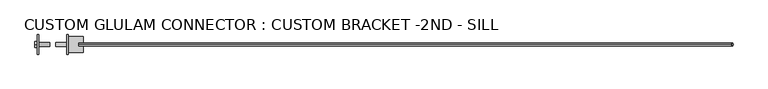
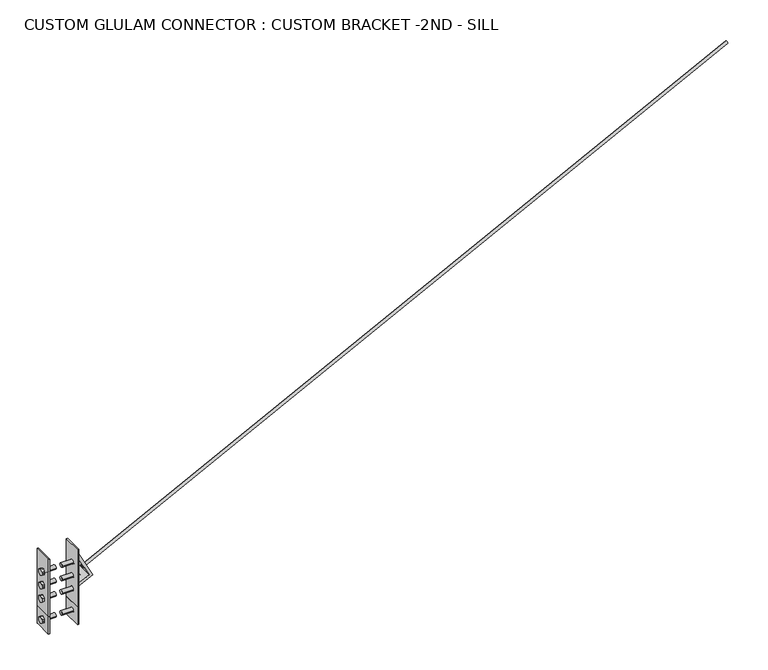
"""IFC4 building model written with IfcOpenShell, lengths in millimetres: fastener geometry, CUSTOM GLULAM CONNECTOR : CUSTOM BRACKET -2ND - SILL."""

from ifc_helpers import new_model, si_unit, point, frame, frame_2d, origin, place, context, project, spatial, polyline, circle_curve, trimmed, segment, composite_curve, outline, extrude, source, transform, mapped, element, save
from ifc_brep_helpers import plane_surface, revolved_surface, advanced_brep


def custom_glulam_connector_custom_bracket_2nd_sill_58b813d6(model_context):
    return source(origin(), model_context, "Body", "SolidModel", [
        advanced_brep(
        [(-95.25, -60.325, 122.2375), (-87.3125, -60.325, 122.2375), (-87.3125, 60.325, 122.2375), (-95.25, 60.325, 122.2375), (-95.25, 52.3875, 122.2375), (-95.25, -60.325, 7.9375), (-87.3125, -60.325, 7.9375), (-95.25, -13.890625, 71.4375), (-95.25, 13.890625, 71.4375), (-87.3125, 13.890625, 71.4375), (-87.3125, -13.890625, 71.4375), (-95.25, 60.325, 7.9375), (-95.25, 52.3875, 7.9375), (-87.3125, 60.325, 7.9375)],
        [
            (0, 1),
            (1, 2),
            (2, 3),
            (3, 4),
            (4, 0),
            (5, 6),
            (6, 1),
            (0, 5),
            (7, 8, circle_curve(frame((-95.25, 0.0, 71.4375), z_axis=(-1.0, 0.0, 0.0), x_axis=(0.0, 1.0, 0.0)), 13.890625)),
            (8, 9),
            (9, 10, circle_curve(frame((-87.3125, 0.0, 71.4375), z_axis=(1.0, 0.0, 0.0), x_axis=(0.0, 1.0, 0.0)), 13.890625)),
            (10, 7),
            (3, 11),
            (11, 12),
            (12, 5),
            (7, 8, circle_curve(frame((-95.25, 0.0, 71.4375), z_axis=(1.0, 0.0, 0.0), x_axis=(0.0, 1.0, 0.0)), 13.890625)),
            (2, 13),
            (13, 11),
            (10, 9, circle_curve(frame((-87.3125, 0.0, 71.4375), z_axis=(1.0, 0.0, 0.0), x_axis=(0.0, 1.0, 0.0)), 13.890625)),
            (6, 13),
        ],
        [
            plane_surface(frame((-95.25, 60.325, 122.2375), z_axis=(0.0, 0.0, 1.0), x_axis=(1.0, 0.0, 0.0))),
            plane_surface(frame((-95.25, -60.325, 122.2375), z_axis=(0.0, -1.0, 0.0), x_axis=(1.0, 0.0, 0.0))),
            revolved_surface(polyline([(-95.25, 13.890625, 71.4375), (-87.3125, 13.890625, 71.4375)]), (-87.3125, 0.0, 71.4375), (-1.0, 0.0, 0.0)),
            plane_surface(frame((-95.25, -60.325, 122.2375), z_axis=(-1.0, 0.0, 0.0), x_axis=(0.0, -1.0, 0.0))),
            plane_surface(frame((-95.25, 60.325, 7.9375), z_axis=(0.0, 1.0, 0.0), x_axis=(1.0, 0.0, 0.0))),
            plane_surface(frame((-87.3125, -60.325, 122.2375), z_axis=(1.0, 0.0, 0.0), x_axis=(0.0, 1.0, 0.0))),
            plane_surface(frame((-95.25, -60.325, 7.9375), z_axis=(0.0, 0.0, -1.0), x_axis=(1.0, 0.0, 0.0))),
        ],
        [
            (0, [[1, 2, 3, 4, 5]]),
            (1, [[6, 7, -1, 8]]),
            (2, [[9, 10, 11, 12]]),
            (3, [[13, 14, 15, -8, -5, -4], [-9, 16]]),
            (4, [[-3, 17, 18, -13]]),
            (2, [[19, -10, -16, -12]]),
            (5, [[-2, -7, 20, -17], [-11, -19]]),
            (6, [[-18, -20, -6, -15, -14]]),
        ],
    ),
        extrude(outline(polyline([(-19.05, 82.4360226), (0.0, 93.4345453), (19.05, 82.4360226), (19.05, 60.4389774), (0.0, 49.4404547), (-19.05, 60.4389774), (-19.05, 82.4360226)])), frame((-110.2320312, 0.0, 0.0), z_axis=(1.0, 0.0, 0.0), x_axis=(0.0, 1.0, 0.0)), (0.0, 0.0, 1.0), 14.9820312),
        extrude(outline(composite_curve([segment(trimmed(circle_curve(frame_2d((0.0, 71.4375)), 12.7), [point((-12.7, 71.4375))], [point((12.7, 71.4375))], False, "CARTESIAN"), True, "CONTINUOUS"), segment(trimmed(circle_curve(frame_2d((0.0, 71.4375)), 12.7), [point((12.7, 71.4375))], [point((-12.7, 71.4375))], False, "CARTESIAN"), True, "CONTINUOUS")], self_intersect=False)), frame((-95.25, 0.0, 0.0), z_axis=(1.0, 0.0, 0.0), x_axis=(0.0, 1.0, 0.0)), (0.0, 0.0, 1.0), 76.2),
        advanced_brep(
        [(95.25, -60.325, 122.2375), (95.25, 52.3875, 122.2375), (95.25, 60.325, 122.2375), (87.3125, 60.325, 122.2375), (87.3125, -60.325, 122.2375), (95.25, -60.325, 7.9375), (87.3125, -60.325, 7.9375), (95.25, -13.890625, 71.4375), (87.3125, -13.890625, 71.4375), (87.3125, 13.890625, 71.4375), (95.25, 13.890625, 71.4375), (95.25, 52.3875, 7.9375), (95.25, 60.325, 7.9375), (87.3125, 60.325, 7.9375)],
        [
            (0, 1),
            (1, 2),
            (2, 3),
            (3, 4),
            (4, 0),
            (5, 0),
            (4, 6),
            (6, 5),
            (7, 8),
            (8, 9, circle_curve(frame((87.3125, 0.0, 71.4375), z_axis=(-1.0, 0.0, 0.0), x_axis=(0.0, 1.0, 0.0)), 13.890625)),
            (9, 10),
            (10, 7, circle_curve(frame((95.25, 0.0, 71.4375), z_axis=(1.0, 0.0, 0.0), x_axis=(0.0, 1.0, 0.0)), 13.890625)),
            (5, 11),
            (11, 12),
            (12, 2),
            (10, 7, circle_curve(frame((95.25, 0.0, 71.4375), z_axis=(-1.0, 0.0, 0.0), x_axis=(0.0, 1.0, 0.0)), 13.890625)),
            (12, 13),
            (13, 3),
            (9, 8, circle_curve(frame((87.3125, 0.0, 71.4375), z_axis=(-1.0, 0.0, 0.0), x_axis=(0.0, 1.0, 0.0)), 13.890625)),
            (13, 6),
        ],
        [
            plane_surface(frame((95.25, 60.325, 122.2375), z_axis=(0.0, 0.0, 1.0), x_axis=(-1.0, 0.0, 0.0))),
            plane_surface(frame((95.25, -60.325, 122.2375), z_axis=(0.0, -1.0, 0.0), x_axis=(-1.0, 0.0, 0.0))),
            revolved_surface(polyline([(95.25, 13.890625, 71.4375), (87.3125, 13.890625, 71.4375)]), (87.3125, 0.0, 71.4375), (1.0, 0.0, 0.0)),
            plane_surface(frame((95.25, -60.325, 122.2375), z_axis=(1.0, 0.0, 0.0), x_axis=(0.0, -1.0, 0.0))),
            plane_surface(frame((95.25, 60.325, 7.9375), z_axis=(0.0, 1.0, 0.0), x_axis=(-1.0, 0.0, 0.0))),
            plane_surface(frame((87.3125, -60.325, 122.2375), z_axis=(-1.0, 0.0, 0.0), x_axis=(0.0, 1.0, 0.0))),
            plane_surface(frame((95.25, -60.325, 7.9375), z_axis=(0.0, 0.0, -1.0), x_axis=(-1.0, 0.0, 0.0))),
        ],
        [
            (0, [[1, 2, 3, 4, 5]]),
            (1, [[6, -5, 7, 8]]),
            (2, [[9, 10, 11, 12]]),
            (3, [[-2, -1, -6, 13, 14, 15], [16, -12]]),
            (4, [[-15, 17, 18, -3]]),
            (2, [[-9, -16, -11, 19]]),
            (5, [[-18, 20, -7, -4], [-19, -10]]),
            (6, [[-14, -13, -8, -20, -17]]),
        ],
    ),
        extrude(outline(polyline([(-19.05, 82.4360226), (0.0, 93.4345453), (19.05, 82.4360226), (19.05, 60.4389774), (0.0, 49.4404547), (-19.05, 60.4389774), (-19.05, 82.4360226)])), frame((95.25, 0.0, 0.0), z_axis=(1.0, 0.0, 0.0), x_axis=(0.0, 1.0, 0.0)), (0.0, 0.0, 1.0), 14.9820312),
        extrude(outline(composite_curve([segment(trimmed(circle_curve(frame_2d((0.0, 71.4375)), 12.7), [point((-12.7, 71.4375))], [point((12.7, 71.4375))], False, "CARTESIAN"), True, "CONTINUOUS"), segment(trimmed(circle_curve(frame_2d((0.0, 71.4375)), 12.7), [point((12.7, 71.4375))], [point((-12.7, 71.4375))], False, "CARTESIAN"), True, "CONTINUOUS")], self_intersect=False)), frame((19.05, 0.0, 0.0), z_axis=(1.0, 0.0, 0.0), x_axis=(0.0, 1.0, 0.0)), (0.0, 0.0, 1.0), 76.2),
        advanced_brep(
        [(-95.25, 60.325, 503.2375), (-87.3125, 60.325, 503.2375), (-87.3125, 60.325, 122.2375), (-95.25, 60.325, 122.2375), (-87.3125, -13.890625, 388.9375), (-87.3125, 13.890625, 388.9375), (-95.25, 13.890625, 388.9375), (-95.25, -13.890625, 388.9375), (-95.25, -60.325, 503.2375), (-87.3125, -60.325, 503.2375), (-95.25, -52.3875, 503.2375), (-95.25, -52.3875, 122.2375), (-95.25, -60.325, 122.2375), (-95.25, 13.890625, 300.0375), (-95.25, -13.890625, 300.0375), (-95.25, 13.890625, 211.1375), (-95.25, -13.890625, 211.1375), (-87.3125, -13.890625, 300.0375), (-87.3125, 13.890625, 300.0375), (-87.3125, -60.325, 122.2375), (-87.3125, -13.890625, 211.1375), (-87.3125, 13.890625, 211.1375)],
        [
            (0, 1),
            (1, 2),
            (2, 3),
            (3, 0),
            (4, 5, circle_curve(frame((-87.3125, 0.0, 388.9375), z_axis=(1.0, 0.0, 0.0), x_axis=(0.0, 1.0, 0.0)), 13.890625)),
            (5, 6),
            (6, 7, circle_curve(frame((-95.25, 0.0, 388.9375), z_axis=(-1.0, 0.0, 0.0), x_axis=(0.0, 1.0, 0.0)), 13.890625)),
            (7, 4),
            (7, 6, circle_curve(frame((-95.25, 0.0, 388.9375), z_axis=(-1.0, 0.0, 0.0), x_axis=(0.0, 1.0, 0.0)), 13.890625)),
            (5, 4, circle_curve(frame((-87.3125, 0.0, 388.9375), z_axis=(1.0, 0.0, 0.0), x_axis=(0.0, 1.0, 0.0)), 13.890625)),
            (8, 9),
            (9, 1),
            (0, 10),
            (10, 8),
            (3, 11),
            (11, 12),
            (12, 8),
            (13, 14, circle_curve(frame((-95.25, 0.0, 300.0375), z_axis=(1.0, 0.0, 0.0), x_axis=(0.0, 1.0, 0.0)), 13.890625)),
            (14, 13, circle_curve(frame((-95.25, 0.0, 300.0375), z_axis=(1.0, 0.0, 0.0), x_axis=(0.0, 1.0, 0.0)), 13.890625)),
            (15, 16, circle_curve(frame((-95.25, 0.0, 211.1375), z_axis=(1.0, 0.0, 0.0), x_axis=(0.0, 1.0, 0.0)), 13.890625)),
            (16, 15, circle_curve(frame((-95.25, 0.0, 211.1375), z_axis=(1.0, 0.0, 0.0), x_axis=(0.0, 1.0, 0.0)), 13.890625)),
            (17, 18, circle_curve(frame((-87.3125, 0.0, 300.0375), z_axis=(1.0, 0.0, 0.0), x_axis=(0.0, 1.0, 0.0)), 13.890625)),
            (18, 13),
            (14, 17),
            (18, 17, circle_curve(frame((-87.3125, 0.0, 300.0375), z_axis=(1.0, 0.0, 0.0), x_axis=(0.0, 1.0, 0.0)), 13.890625)),
            (9, 19),
            (19, 2),
            (20, 21, circle_curve(frame((-87.3125, 0.0, 211.1375), z_axis=(-1.0, 0.0, 0.0), x_axis=(0.0, 1.0, 0.0)), 13.890625)),
            (21, 20, circle_curve(frame((-87.3125, 0.0, 211.1375), z_axis=(-1.0, 0.0, 0.0), x_axis=(0.0, 1.0, 0.0)), 13.890625)),
            (12, 19),
            (21, 15),
            (16, 20),
        ],
        [
            plane_surface(frame((-95.25, 60.325, 122.2375), z_axis=(0.0, 1.0, 0.0), x_axis=(1.0, 0.0, 0.0))),
            revolved_surface(polyline([(-95.25, 13.890625, 388.9375), (-87.3125, 13.890625, 388.9375)]), (-87.3125, 0.0, 388.9375), (-1.0, 0.0, 0.0)),
            plane_surface(frame((-95.25, 60.325, 503.2375), z_axis=(0.0, 0.0, 1.0), x_axis=(1.0, 0.0, 0.0))),
            plane_surface(frame((-95.25, -60.325, 503.2375), z_axis=(-1.0, 0.0, 0.0), x_axis=(0.0, -1.0, 0.0))),
            revolved_surface(polyline([(-95.25, 13.890625, 300.0375), (-87.3125, 13.890625, 300.0375)]), (-87.3125, 0.0, 300.0375), (-1.0, 0.0, 0.0)),
            plane_surface(frame((-87.3125, -60.325, 503.2375), z_axis=(1.0, 0.0, 0.0), x_axis=(0.0, 1.0, 0.0))),
            plane_surface(frame((-95.25, -60.325, 503.2375), z_axis=(0.0, -1.0, 0.0), x_axis=(1.0, 0.0, 0.0))),
            plane_surface(frame((-95.25, -60.325, 122.2375), z_axis=(0.0, 0.0, -1.0), x_axis=(1.0, 0.0, 0.0))),
            revolved_surface(polyline([(-95.25, 13.890625, 211.1375), (-87.3125, 13.890625, 211.1375)]), (-87.3125, 0.0, 211.1375), (-1.0, 0.0, 0.0)),
        ],
        [
            (0, [[1, 2, 3, 4]]),
            (1, [[5, 6, 7, 8]]),
            (1, [[9, -6, 10, -8]]),
            (2, [[11, 12, -1, 13, 14]]),
            (3, [[-4, 15, 16, 17, -14, -13], [18, 19], [-9, -7], [20, 21]]),
            (4, [[22, 23, -19, 24]]),
            (4, [[-18, -23, 25, -24]]),
            (5, [[-12, 26, 27, -2], [-10, -5], [-25, -22], [28, 29]]),
            (6, [[30, -26, -11, -17]]),
            (7, [[-3, -27, -30, -16, -15]]),
            (8, [[-29, 31, -21, 32]]),
            (8, [[-20, -31, -28, -32]]),
        ],
    ),
        extrude(outline(polyline([(-19.05, 399.9360226), (0.0, 410.9345453), (19.05, 399.9360226), (19.05, 377.9389774), (0.0, 366.9404547), (-19.05, 377.9389774), (-19.05, 399.9360226)])), frame((-110.2320312, 0.0, 0.0), z_axis=(1.0, 0.0, 0.0), x_axis=(0.0, 1.0, 0.0)), (0.0, 0.0, 1.0), 14.9820312),
        extrude(outline(composite_curve([segment(trimmed(circle_curve(frame_2d((0.0, 388.9375)), 12.7), [point((-12.7, 388.9375))], [point((12.7, 388.9375))], False, "CARTESIAN"), True, "CONTINUOUS"), segment(trimmed(circle_curve(frame_2d((0.0, 388.9375)), 12.7), [point((12.7, 388.9375))], [point((-12.7, 388.9375))], False, "CARTESIAN"), True, "CONTINUOUS")], self_intersect=False)), frame((-95.25, 0.0, 0.0), z_axis=(1.0, 0.0, 0.0), x_axis=(0.0, 1.0, 0.0)), (0.0, 0.0, 1.0), 76.2),
        extrude(outline(polyline([(-19.05, 311.0360226), (0.0, 322.0345453), (19.05, 311.0360226), (19.05, 289.0389774), (0.0, 278.0404547), (-19.05, 289.0389774), (-19.05, 311.0360226)])), frame((-110.2320312, 0.0, 0.0), z_axis=(1.0, 0.0, 0.0), x_axis=(0.0, 1.0, 0.0)), (0.0, 0.0, 1.0), 14.9820312),
        extrude(outline(composite_curve([segment(trimmed(circle_curve(frame_2d((0.0, 300.0375)), 12.7), [point((-12.7, 300.0375))], [point((12.7, 300.0375))], False, "CARTESIAN"), True, "CONTINUOUS"), segment(trimmed(circle_curve(frame_2d((0.0, 300.0375)), 12.7), [point((12.7, 300.0375))], [point((-12.7, 300.0375))], False, "CARTESIAN"), True, "CONTINUOUS")], self_intersect=False)), frame((-95.25, 0.0, 0.0), z_axis=(1.0, 0.0, 0.0), x_axis=(0.0, 1.0, 0.0)), (0.0, 0.0, 1.0), 76.2),
        extrude(outline(polyline([(-19.05, 399.9360226), (0.0, 410.9345453), (19.05, 399.9360226), (19.05, 377.9389774), (0.0, 366.9404547), (-19.05, 377.9389774), (-19.05, 399.9360226)])), frame((-110.2320312, 0.0, 0.0), z_axis=(1.0, 0.0, 0.0), x_axis=(0.0, 1.0, 0.0)), (0.0, 0.0, 1.0), 14.9820312),
        extrude(outline(composite_curve([segment(trimmed(circle_curve(frame_2d((0.0, 388.9375)), 12.7), [point((-12.7, 388.9375))], [point((12.7, 388.9375))], False, "CARTESIAN"), True, "CONTINUOUS"), segment(trimmed(circle_curve(frame_2d((0.0, 388.9375)), 12.7), [point((12.7, 388.9375))], [point((-12.7, 388.9375))], False, "CARTESIAN"), True, "CONTINUOUS")], self_intersect=False)), frame((-95.25, 0.0, 0.0), z_axis=(1.0, 0.0, 0.0), x_axis=(0.0, 1.0, 0.0)), (0.0, 0.0, 1.0), 76.2),
        extrude(outline(polyline([(-19.05, 222.1360226), (0.0, 233.1345453), (19.05, 222.1360226), (19.05, 200.1389774), (0.0, 189.1404547), (-19.05, 200.1389774), (-19.05, 222.1360226)])), frame((-110.2320312, 0.0, 0.0), z_axis=(1.0, 0.0, 0.0), x_axis=(0.0, 1.0, 0.0)), (0.0, 0.0, 1.0), 14.9820312),
        extrude(outline(composite_curve([segment(trimmed(circle_curve(frame_2d((0.0, 211.1375)), 12.7), [point((-12.7, 211.1375))], [point((12.7, 211.1375))], False, "CARTESIAN"), True, "CONTINUOUS"), segment(trimmed(circle_curve(frame_2d((0.0, 211.1375)), 12.7), [point((12.7, 211.1375))], [point((-12.7, 211.1375))], False, "CARTESIAN"), True, "CONTINUOUS")], self_intersect=False)), frame((-95.25, 0.0, 0.0), z_axis=(1.0, 0.0, 0.0), x_axis=(0.0, 1.0, 0.0)), (0.0, 0.0, 1.0), 76.2),
        advanced_brep(
        [(95.25, 60.325, 503.2375), (95.25, 60.325, 122.2375), (87.3125, 60.325, 122.2375), (87.3125, 60.325, 503.2375), (87.3125, -13.890625, 388.9375), (95.25, -13.890625, 388.9375), (95.25, 13.890625, 388.9375), (87.3125, 13.890625, 388.9375), (95.25, -60.325, 503.2375), (95.25, -52.3875, 503.2375), (87.3125, -60.325, 503.2375), (95.25, -60.325, 122.2375), (95.25, -52.3875, 122.2375), (95.25, 13.890625, 300.0375), (95.25, -13.890625, 300.0375), (95.25, 13.890625, 211.1375), (95.25, -13.890625, 211.1375), (87.3125, -13.890625, 300.0375), (87.3125, 13.890625, 300.0375), (87.3125, -60.325, 122.2375), (87.3125, -13.890625, 211.1375), (87.3125, 13.890625, 211.1375)],
        [
            (0, 1),
            (1, 2),
            (2, 3),
            (3, 0),
            (4, 5),
            (5, 6, circle_curve(frame((95.25, 0.0, 388.9375), z_axis=(1.0, 0.0, 0.0), x_axis=(0.0, 1.0, 0.0)), 13.890625)),
            (6, 7),
            (7, 4, circle_curve(frame((87.3125, 0.0, 388.9375), z_axis=(-1.0, 0.0, 0.0), x_axis=(0.0, 1.0, 0.0)), 13.890625)),
            (4, 7, circle_curve(frame((87.3125, 0.0, 388.9375), z_axis=(-1.0, 0.0, 0.0), x_axis=(0.0, 1.0, 0.0)), 13.890625)),
            (6, 5, circle_curve(frame((95.25, 0.0, 388.9375), z_axis=(1.0, 0.0, 0.0), x_axis=(0.0, 1.0, 0.0)), 13.890625)),
            (8, 9),
            (9, 0),
            (3, 10),
            (10, 8),
            (8, 11),
            (11, 12),
            (12, 1),
            (13, 14, circle_curve(frame((95.25, 0.0, 300.0375), z_axis=(-1.0, 0.0, 0.0), x_axis=(0.0, 1.0, 0.0)), 13.890625)),
            (14, 13, circle_curve(frame((95.25, 0.0, 300.0375), z_axis=(-1.0, 0.0, 0.0), x_axis=(0.0, 1.0, 0.0)), 13.890625)),
            (15, 16, circle_curve(frame((95.25, 0.0, 211.1375), z_axis=(-1.0, 0.0, 0.0), x_axis=(0.0, 1.0, 0.0)), 13.890625)),
            (16, 15, circle_curve(frame((95.25, 0.0, 211.1375), z_axis=(-1.0, 0.0, 0.0), x_axis=(0.0, 1.0, 0.0)), 13.890625)),
            (17, 14),
            (13, 18),
            (18, 17, circle_curve(frame((87.3125, 0.0, 300.0375), z_axis=(-1.0, 0.0, 0.0), x_axis=(0.0, 1.0, 0.0)), 13.890625)),
            (17, 18, circle_curve(frame((87.3125, 0.0, 300.0375), z_axis=(-1.0, 0.0, 0.0), x_axis=(0.0, 1.0, 0.0)), 13.890625)),
            (2, 19),
            (19, 10),
            (20, 21, circle_curve(frame((87.3125, 0.0, 211.1375), z_axis=(1.0, 0.0, 0.0), x_axis=(0.0, 1.0, 0.0)), 13.890625)),
            (21, 20, circle_curve(frame((87.3125, 0.0, 211.1375), z_axis=(1.0, 0.0, 0.0), x_axis=(0.0, 1.0, 0.0)), 13.890625)),
            (19, 11),
            (20, 16),
            (15, 21),
        ],
        [
            plane_surface(frame((95.25, 60.325, 122.2375), z_axis=(0.0, 1.0, 0.0), x_axis=(-1.0, 0.0, 0.0))),
            revolved_surface(polyline([(95.25, 13.890625, 388.9375), (87.3125, 13.890625, 388.9375)]), (87.3125, 0.0, 388.9375), (1.0, 0.0, 0.0)),
            plane_surface(frame((95.25, 60.325, 503.2375), z_axis=(0.0, 0.0, 1.0), x_axis=(-1.0, 0.0, 0.0))),
            plane_surface(frame((95.25, -60.325, 503.2375), z_axis=(1.0, 0.0, 0.0), x_axis=(0.0, -1.0, 0.0))),
            revolved_surface(polyline([(95.25, 13.890625, 300.0375), (87.3125, 13.890625, 300.0375)]), (87.3125, 0.0, 300.0375), (1.0, 0.0, 0.0)),
            plane_surface(frame((87.3125, -60.325, 503.2375), z_axis=(-1.0, 0.0, 0.0), x_axis=(0.0, 1.0, 0.0))),
            plane_surface(frame((95.25, -60.325, 503.2375), z_axis=(0.0, -1.0, 0.0), x_axis=(-1.0, 0.0, 0.0))),
            plane_surface(frame((95.25, -60.325, 122.2375), z_axis=(0.0, 0.0, -1.0), x_axis=(-1.0, 0.0, 0.0))),
            revolved_surface(polyline([(95.25, 13.890625, 211.1375), (87.3125, 13.890625, 211.1375)]), (87.3125, 0.0, 211.1375), (1.0, 0.0, 0.0)),
        ],
        [
            (0, [[1, 2, 3, 4]]),
            (1, [[5, 6, 7, 8]]),
            (1, [[-5, 9, -7, 10]]),
            (2, [[11, 12, -4, 13, 14]]),
            (3, [[-12, -11, 15, 16, 17, -1], [-6, -10], [18, 19], [20, 21]]),
            (4, [[22, -18, 23, 24]]),
            (4, [[-22, 25, -23, -19]]),
            (5, [[-3, 26, 27, -13], [-8, -9], [-24, -25], [28, 29]]),
            (6, [[-15, -14, -27, 30]]),
            (7, [[-17, -16, -30, -26, -2]]),
            (8, [[31, -20, 32, -28]]),
            (8, [[-31, -29, -32, -21]]),
        ],
    ),
        extrude(outline(polyline([(-19.05, 399.9360226), (0.0, 410.9345453), (19.05, 399.9360226), (19.05, 377.9389774), (0.0, 366.9404547), (-19.05, 377.9389774), (-19.05, 399.9360226)])), frame((95.25, 0.0, 0.0), z_axis=(1.0, 0.0, 0.0), x_axis=(0.0, 1.0, 0.0)), (0.0, 0.0, 1.0), 14.9820312),
        extrude(outline(composite_curve([segment(trimmed(circle_curve(frame_2d((0.0, 388.9375)), 12.7), [point((-12.7, 388.9375))], [point((12.7, 388.9375))], False, "CARTESIAN"), True, "CONTINUOUS"), segment(trimmed(circle_curve(frame_2d((0.0, 388.9375)), 12.7), [point((12.7, 388.9375))], [point((-12.7, 388.9375))], False, "CARTESIAN"), True, "CONTINUOUS")], self_intersect=False)), frame((19.05, 0.0, 0.0), z_axis=(1.0, 0.0, 0.0), x_axis=(0.0, 1.0, 0.0)), (0.0, 0.0, 1.0), 76.2),
        extrude(outline(polyline([(-19.05, 311.0360226), (0.0, 322.0345453), (19.05, 311.0360226), (19.05, 289.0389774), (0.0, 278.0404547), (-19.05, 289.0389774), (-19.05, 311.0360226)])), frame((95.25, 0.0, 0.0), z_axis=(1.0, 0.0, 0.0), x_axis=(0.0, 1.0, 0.0)), (0.0, 0.0, 1.0), 14.9820312),
        extrude(outline(composite_curve([segment(trimmed(circle_curve(frame_2d((0.0, 300.0375)), 12.7), [point((-12.7, 300.0375))], [point((12.7, 300.0375))], False, "CARTESIAN"), True, "CONTINUOUS"), segment(trimmed(circle_curve(frame_2d((0.0, 300.0375)), 12.7), [point((12.7, 300.0375))], [point((-12.7, 300.0375))], False, "CARTESIAN"), True, "CONTINUOUS")], self_intersect=False)), frame((19.05, 0.0, 0.0), z_axis=(1.0, 0.0, 0.0), x_axis=(0.0, 1.0, 0.0)), (0.0, 0.0, 1.0), 76.2),
        extrude(outline(polyline([(-19.05, 399.9360226), (0.0, 410.9345453), (19.05, 399.9360226), (19.05, 377.9389774), (0.0, 366.9404547), (-19.05, 377.9389774), (-19.05, 399.9360226)])), frame((95.25, 0.0, 0.0), z_axis=(1.0, 0.0, 0.0), x_axis=(0.0, 1.0, 0.0)), (0.0, 0.0, 1.0), 14.9820312),
        extrude(outline(composite_curve([segment(trimmed(circle_curve(frame_2d((0.0, 388.9375)), 12.7), [point((-12.7, 388.9375))], [point((12.7, 388.9375))], False, "CARTESIAN"), True, "CONTINUOUS"), segment(trimmed(circle_curve(frame_2d((0.0, 388.9375)), 12.7), [point((12.7, 388.9375))], [point((-12.7, 388.9375))], False, "CARTESIAN"), True, "CONTINUOUS")], self_intersect=False)), frame((19.05, 0.0, 0.0), z_axis=(1.0, 0.0, 0.0), x_axis=(0.0, 1.0, 0.0)), (0.0, 0.0, 1.0), 76.2),
        extrude(outline(polyline([(-19.05, 222.1360226), (0.0, 233.1345453), (19.05, 222.1360226), (19.05, 200.1389774), (0.0, 189.1404547), (-19.05, 200.1389774), (-19.05, 222.1360226)])), frame((95.25, 0.0, 0.0), z_axis=(1.0, 0.0, 0.0), x_axis=(0.0, 1.0, 0.0)), (0.0, 0.0, 1.0), 14.9820312),
        extrude(outline(composite_curve([segment(trimmed(circle_curve(frame_2d((0.0, 211.1375)), 12.7), [point((-12.7, 211.1375))], [point((12.7, 211.1375))], False, "CARTESIAN"), True, "CONTINUOUS"), segment(trimmed(circle_curve(frame_2d((0.0, 211.1375)), 12.7), [point((12.7, 211.1375))], [point((-12.7, 211.1375))], False, "CARTESIAN"), True, "CONTINUOUS")], self_intersect=False)), frame((19.05, 0.0, 0.0), z_axis=(1.0, 0.0, 0.0), x_axis=(0.0, 1.0, 0.0)), (0.0, 0.0, 1.0), 76.2),
        extrude(outline(composite_curve([segment(trimmed(circle_curve(frame_2d((0.0, -9.525)), 9.525), [point((0.0, -19.05))], [point((0.0, 0.0))], False, "CARTESIAN"), True, "CONTINUOUS"), segment(trimmed(circle_curve(frame_2d((0.0, -9.525)), 9.525), [point((0.0, 0.0))], [point((0.0, -19.05))], False, "CARTESIAN"), True, "CONTINUOUS")], self_intersect=False)), frame((168.4522778, 0.0, 334.447439), z_axis=(0.8910065241883687, 0.0, 0.45399049973954547), x_axis=(0.0, -1.0, 0.0)), (0.0, 0.0, 1.0), 4521.2),
        advanced_brep(
        [(187.1907357, -50.8, 297.6711447), (95.25, -50.8, 478.1149985), (95.25, -50.8, 443.1473064), (165.838908, -50.8, 304.6087741), (95.25, -50.8, 268.641929), (95.25, -50.8, 250.825), (187.1907357, 50.8, 297.6711447), (95.25, 50.8, 250.825), (95.25, 50.8, 268.641929), (165.838908, 50.8, 304.6087741), (95.25, 50.8, 443.1473064), (95.25, 50.8, 478.1149985), (168.9928103, 0.0, 333.3865843), (159.2632264, 0.0, 352.4819679), (145.1184978, 0.0, 345.2748687), (154.8480817, 0.0, 326.1794852), (135.0741233, 0.0, 288.9333334), (134.3668869, 0.0, 288.5729784), (141.5739861, 0.0, 274.4282498), (142.2812225, 0.0, 274.7886048)],
        [
            (0, 1),
            (1, 2),
            (2, 3),
            (3, 4),
            (4, 5),
            (5, 0),
            (6, 7),
            (7, 8),
            (8, 9),
            (9, 10),
            (10, 11),
            (11, 6),
            (0, 6),
            (11, 1),
            (12, 13, circle_curve(frame((164.1280183, 0.0, 342.9342761), z_axis=(-0.8910065241883687, 0.0, -0.45399049973954547), x_axis=(-0.45399049973954547, 0.0, 0.8910065241883687)), 10.715625)),
            (13, 12, circle_curve(frame((164.1280183, 0.0, 342.9342761), z_axis=(-0.8910065241883687, 0.0, -0.45399049973954547), x_axis=(-0.45399049973954547, 0.0, 0.8910065241883687)), 10.715625)),
            (10, 2),
            (9, 3),
            (14, 15, circle_curve(frame((149.9832898, 0.0, 335.7271769), z_axis=(0.8910065241883687, 0.0, 0.45399049973954547), x_axis=(-0.45399049973954547, 0.0, 0.8910065241883687)), 10.715625)),
            (15, 14, circle_curve(frame((149.9832898, 0.0, 335.7271769), z_axis=(0.8910065241883687, 0.0, 0.45399049973954547), x_axis=(-0.45399049973954547, 0.0, 0.8910065241883687)), 10.715625)),
            (8, 4),
            (16, 17, circle_curve(frame((134.7205051, 0.0, 288.7531559), z_axis=(0.4539904997395443, 0.0, -0.8910065241883692), x_axis=(0.8910065241883692, 0.0, 0.4539904997395443)), 0.396875)),
            (17, 16, circle_curve(frame((134.7205051, 0.0, 288.7531559), z_axis=(0.4539904997395443, 0.0, -0.8910065241883692), x_axis=(0.8910065241883692, 0.0, 0.4539904997395443)), 0.396875)),
            (7, 5),
            (18, 19, circle_curve(frame((141.9276043, 0.0, 274.6084273), z_axis=(-0.4539904997395443, 0.0, 0.8910065241883692), x_axis=(0.8910065241883692, 0.0, 0.4539904997395443)), 0.396875)),
            (19, 18, circle_curve(frame((141.9276043, 0.0, 274.6084273), z_axis=(-0.4539904997395443, 0.0, 0.8910065241883692), x_axis=(0.8910065241883692, 0.0, 0.4539904997395443)), 0.396875)),
            (12, 15),
            (14, 13),
            (18, 17),
            (16, 19),
        ],
        [
            plane_surface(frame((95.25, -50.8, 478.1149985), z_axis=(0.0, -1.0000000000000002, 0.0), x_axis=(-0.45399049973954547, 0.0, 0.8910065241883687))),
            plane_surface(frame((95.25, 50.8, 478.1149985), z_axis=(0.0, 1.0000000000000002, 0.0), x_axis=(0.45399049973954547, 0.0, -0.8910065241883687))),
            plane_surface(frame((187.1907357, -50.8, 297.6711447), z_axis=(0.8910065241883687, 0.0, 0.45399049973954547), x_axis=(0.0, 1.0, 0.0))),
            plane_surface(frame((95.25, -50.8, 478.1149985), z_axis=(-1.0, 0.0, 0.0), x_axis=(0.0, 1.0, 0.0))),
            plane_surface(frame((95.25, -50.8, 443.1473064), z_axis=(-0.8910065241883683, 0.0, -0.4539904997395459), x_axis=(0.0, 1.0, 0.0))),
            plane_surface(frame((165.838908, -50.8, 304.6087741), z_axis=(-0.45399049973954425, 0.0, 0.8910065241883692), x_axis=(0.0, 1.0, 0.0))),
            plane_surface(frame((95.25, -50.8, 268.641929), z_axis=(-1.0, 0.0, 0.0), x_axis=(0.0, 1.0, 0.0))),
            plane_surface(frame((95.25, -50.8, 250.825), z_axis=(0.45399049973954425, 0.0, -0.8910065241883692), x_axis=(0.0, 1.0, 0.0))),
            revolved_surface(polyline([(145.1184977948568, 0.0, 345.2748687100941), (159.26322639570964, 0.0, 352.4819679084203)]), (164.1280183, 0.0, 342.9342761), (-0.8910065241883687, 0.0, -0.45399049973954547)),
            revolved_surface(polyline([(135.07412330475796, 0.0, 288.9333334024243), (142.28122252549036, 0.0, 274.78860475759683)]), (141.9276043, 0.0, 274.6084273), (-0.4539904997395443, 0.0, 0.8910065241883692)),
        ],
        [
            (0, [[1, 2, 3, 4, 5, 6]]),
            (1, [[7, 8, 9, 10, 11, 12]]),
            (2, [[-1, 13, -12, 14], [15, 16]]),
            (3, [[-2, -14, -11, 17]]),
            (4, [[-3, -17, -10, 18], [19, 20]]),
            (5, [[-4, -18, -9, 21], [22, 23]]),
            (6, [[-5, -21, -8, 24]]),
            (7, [[-6, -24, -7, -13], [25, 26]]),
            (8, [[27, -19, 28, -15]]),
            (8, [[-27, -16, -28, -20]]),
            (9, [[29, -22, 30, -25]]),
            (9, [[-29, -26, -30, -23]]),
        ],
    ),
    ])


if __name__ == "__main__":
    model = new_model("IFC4")
    model_context = context("Model", 3, world=origin())
    ifc_project = project(units=[si_unit("LENGTHUNIT", "METRE", prefix="MILLI")], contexts=[model_context])
    site = spatial("IfcSite", under=ifc_project)
    building = spatial("IfcBuilding", under=site)
    placement = place(None, origin())
    custom_glulam_connector_custom_bracket_2nd_sill_shape = custom_glulam_connector_custom_bracket_2nd_sill_58b813d6(model_context)
    element("IfcFastener", 1, ObjectType="CUSTOM GLULAM CONNECTOR : CUSTOM BRACKET -2ND - SILL", at=placement, inside=building, context=model_context, shape_type="MappedRepresentation", body=[
        mapped(custom_glulam_connector_custom_bracket_2nd_sill_shape, transform((0.0, 0.0, 0.0), x_axis=(1.0, 0.0, 0.0), y_axis=(0.0, 1.0, 0.0), z_axis=(0.0, 0.0, 1.0))),
    ])
    save(model, "model.ifc")

# Revit data of these elements
# Type "CUSTOM GLULAM CONNECTOR : CUSTOM BRACKET -2ND - SILL"
#   Width - Top = 0' - 6 7/8"
#   Top/Bottom Plate Thickness = 0' - 0 5/16"
#   Top/Bottom Plate - Width = 0' - 7 1/2"
#   Rod Radius = 0' - 0 3/8"
#   Rod Length [instance default] = 1' - 0"
#   Plate Thickness = 0' - 0 5/16"
#   Offset - Upper Plate 2 = 0' - 0"
#   Height of Plate = 0' - 4 1/2"
#   Width - Bottom = 0' - 6 7/8"
#   Plate Width = 0' - 4 3/4"
#   Bracket Width = 0' - 4"
#   Bracket Thickness = 0' - 0 5/8"
#   Bracket Offset in X = 0' - 3 3/4"
#   Bracket Offset in Y = 0' - 0 3/8"
#   Bracket Offset = 0' - 9 7/8"
#   Bracket Leg = 0' - 4 1/16"
#   Bracket Hole Radius - Up = 0' - 0 27/64"
#   Bracket Hole Radius - Down = 0' - 0 1/64"
#   Bracket Hole Offset = 0' - 2"
#   Beam Width = 0' - 7 3/8"
#   Angle 2 = 27.00°
#   Angle 1 = 117.00°
#   Top Plate Visible = no
#   Rod Visibility = yes
#   Plate Visibility - Upper Right 2 = no
#   Plate Visibility - Upper Right 1 = yes
#   Plate Visibility - Upper Left 2 = no
#   Plate Visibility - Upper Left 1 = yes
#   Plate Visibility - Lower Right 2 = no
#   Plate Visibility - Lower Right 1 = yes
#   Plate Visibility - Lower Left 2 = no
#   Plate Visibility - Lower Left 1 = yes
#   Bracket Visibility = yes
#   Bottom Plate Visible = no
#   Upper Plates - 2 = element 1222094
#   Upper Plates - 1 = element 1222094
#   Lower Plates = element 1222095
#   Bracket Material = 5/8" STEEL ANGLE (HDG AFTER FABRICATION)
#   URL = ""
# Element 1 (IfcFastener, "CUSTOM GLULAM CONNECTOR : CUSTOM BRACKET -2ND - SILL")
#   Rod Length = 14' - 10"
#   Materials on its faces: "1\" GALV. LAG BOLT (LENGTH = 1/2\" SHY OF GLULAM DEPTH) -  (GALV. THRU BOLT IF PLATE ON OPP. SIDE OF STRUCT MEMBER)", "5/16\" STEEL PLATE (HDG AFTER FABRICATION)", "5/8\" STEEL ANGLE (HDG AFTER FABRICATION)", "3/4\" GALV. ROD (THREADED AT ENDS) - TURN BUCKLE AT 1/4 POINT OF TOTAL LENGTH"
# Materials
#   "5/8\" STEEL ANGLE (HDG AFTER FABRICATION)": class "Generic", colour RGB 195 195 195, transparency 0, Cost = 0
#   "1\" GALV. LAG BOLT (LENGTH = 1/2\" SHY OF GLULAM DEPTH) -  (GALV. THRU BOLT IF PLATE ON OPP. SIDE OF STRUCT MEMBER)": class "Generic", colour RGB 120 120 120, transparency 0, Cost = 0
#   "5/16\" STEEL PLATE (HDG AFTER FABRICATION)": class "Generic", colour RGB 232 232 232, transparency 0, Cost = 0
#   "3/4\" GALV. ROD (THREADED AT ENDS) - TURN BUCKLE AT 1/4 POINT OF TOTAL LENGTH": class "Generic", colour RGB 120 120 120, transparency 0, Cost = 0
